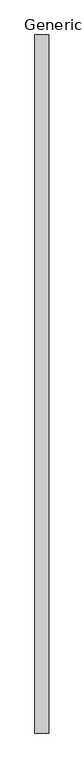
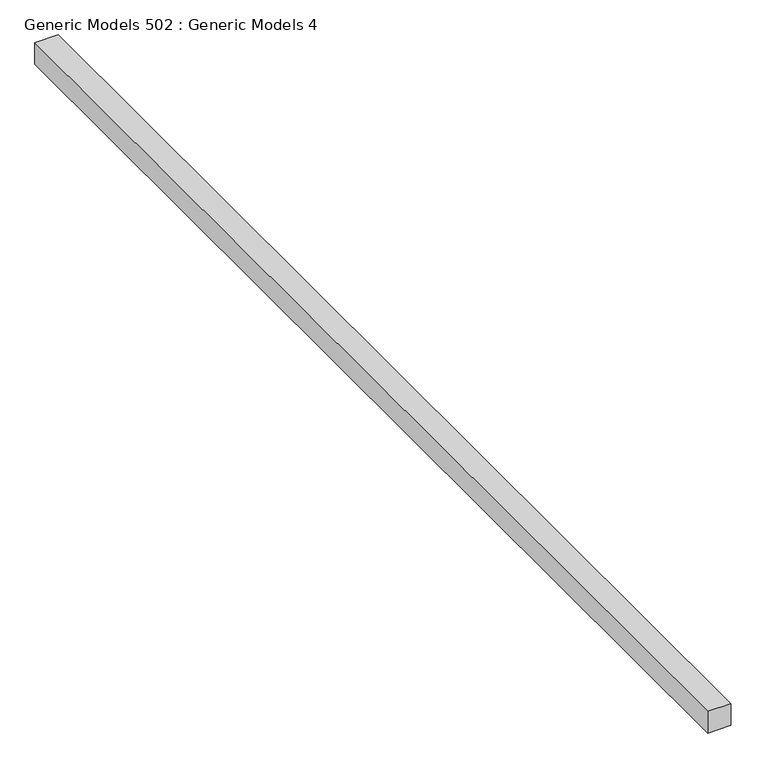
"""IFC4 building model written with IfcOpenShell, lengths in millimetres: proxy geometry, Generic Models 502 : Generic Models 4."""

from ifc_helpers import new_model, si_unit, frame, origin, place, context, project, spatial, polyline, outline, extrude, source, transform, mapped, element, save


def generic_models_502_generic_models_4_4bab93ff(model_context):
    return source(origin(), model_context, "Body", "SweptSolid", [
        extrude(outline(polyline([(-6476.1899522, -6864.9230338), (-6604.7709971, -6864.9230338), (-6604.7709971, -464.1230338), (-6476.1899522, -464.1230338), (-6476.1899522, -6864.9230338)])), frame((0.0, 0.0, 127068.9082912), z_axis=(0.0, 0.0, 1.0), x_axis=(1.0, 0.0, 0.0)), (0.0, 0.0, 1.0), 125.9193991),
    ])


if __name__ == "__main__":
    model = new_model("IFC4")
    model_context = context("Model", 3, world=origin())
    ifc_project = project(units=[si_unit("LENGTHUNIT", "METRE", prefix="MILLI")], contexts=[model_context])
    site = spatial("IfcSite", under=ifc_project)
    building = spatial("IfcBuilding", under=site)
    placement = place(None, origin())
    generic_models_502_generic_models_4_shape = generic_models_502_generic_models_4_4bab93ff(model_context)
    element("IfcBuildingElementProxy", 1, Name="Generic Models 502 : Generic Models 4", ObjectType="Generic Models 502 : Generic Models 4", at=placement, inside=building, context=model_context, shape_type="MappedRepresentation", body=[
        mapped(generic_models_502_generic_models_4_shape, transform((0.0, 0.0, 0.0), x_axis=(1.0, 0.0, 0.0), y_axis=(0.0, 1.0, 0.0), z_axis=(0.0, 0.0, 1.0))),
    ])
    save(model, "model.ifc")

# Revit data of these elements
# Element 1 (IfcBuildingElementProxy, "Generic Models 502 : Generic Models 4")
#   Materials on its faces: "_BATT INSUL. (U-FACTOR = 0.065 MIN.) OVER CLASS II VAPOR RETARDER(TOWARD INTERIOR)"
# Materials
#   "_BATT INSUL. (U-FACTOR = 0.065 MIN.) OVER CLASS II VAPOR RETARDER(TOWARD INTERIOR)": class "Generic", colour RGB 200 166 247, transparency 0, Cost = 0
